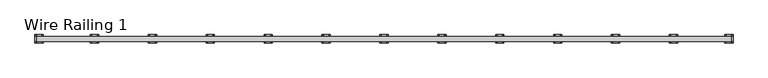
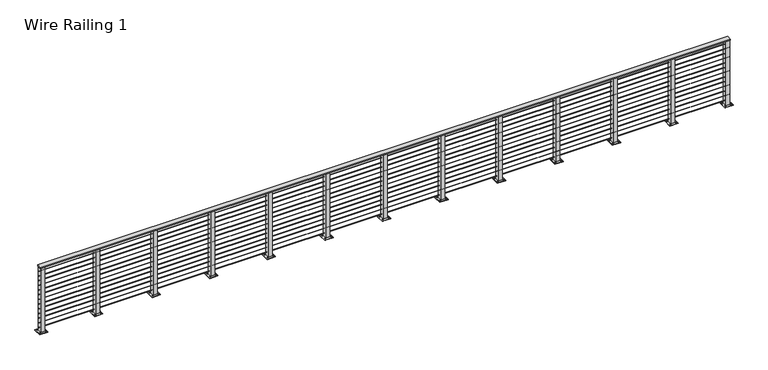
"""IFC4 building model written with IfcOpenShell, lengths in millimetres: railing geometry, Wire Railing 1."""

from ifc_helpers import new_model, si_unit, point, frame, frame_2d, origin, place, context, project, spatial, polyline, circle_curve, trimmed, segment, composite_curve, outline, extrude, source, transform, mapped, element, save


def wire_railing_1_673ce069(model_context):
    return source(origin(), model_context, "Body", "SweptSolid", [
        extrude(outline(polyline([(-281.8532828, -3023.5771465), (-281.8532828, -3099.7771465), (-10899.0532828, -3099.7771465), (-10899.0532828, -3023.5771465), (-281.8532828, -3023.5771465)])), frame((0.0, 0.0, 4502.15), z_axis=(0.0, 0.0, 1.0), x_axis=(1.0, 0.0, 0.0)), (0.0, 0.0, 1.0), 19.05),
        extrude(outline(composite_curve([segment(trimmed(circle_curve(frame_2d((-3061.6771465, 4442.61875)), 2.38125), [point((-3059.2958965, 4442.61875))], [point((-3064.0583965, 4442.61875))], False, "CARTESIAN"), True, "CONTINUOUS"), segment(trimmed(circle_curve(frame_2d((-3061.6771465, 4442.61875)), 2.38125), [point((-3064.0583965, 4442.61875))], [point((-3059.2958965, 4442.61875))], False, "CARTESIAN"), True, "CONTINUOUS")], self_intersect=False)), frame((-10899.0532828, 0.0, 0.0), z_axis=(1.0, 0.0, 0.0), x_axis=(0.0, 1.0, 0.0)), (0.0, 0.0, 1.0), 10617.2),
        extrude(outline(composite_curve([segment(trimmed(circle_curve(frame_2d((-3061.6771465, 4366.41875)), 2.38125), [point((-3059.2958965, 4366.41875))], [point((-3064.0583965, 4366.41875))], False, "CARTESIAN"), True, "CONTINUOUS"), segment(trimmed(circle_curve(frame_2d((-3061.6771465, 4366.41875)), 2.38125), [point((-3064.0583965, 4366.41875))], [point((-3059.2958965, 4366.41875))], False, "CARTESIAN"), True, "CONTINUOUS")], self_intersect=False)), frame((-10899.0532828, 0.0, 0.0), z_axis=(1.0, 0.0, 0.0), x_axis=(0.0, 1.0, 0.0)), (0.0, 0.0, 1.0), 10617.2),
        extrude(outline(composite_curve([segment(trimmed(circle_curve(frame_2d((-3061.6771465, 4290.21875)), 2.38125), [point((-3059.2958965, 4290.21875))], [point((-3064.0583965, 4290.21875))], False, "CARTESIAN"), True, "CONTINUOUS"), segment(trimmed(circle_curve(frame_2d((-3061.6771465, 4290.21875)), 2.38125), [point((-3064.0583965, 4290.21875))], [point((-3059.2958965, 4290.21875))], False, "CARTESIAN"), True, "CONTINUOUS")], self_intersect=False)), frame((-10899.0532828, 0.0, 0.0), z_axis=(1.0, 0.0, 0.0), x_axis=(0.0, 1.0, 0.0)), (0.0, 0.0, 1.0), 10617.2),
        extrude(outline(composite_curve([segment(trimmed(circle_curve(frame_2d((-3061.6771465, 4214.01875)), 2.38125), [point((-3059.2958965, 4214.01875))], [point((-3064.0583965, 4214.01875))], False, "CARTESIAN"), True, "CONTINUOUS"), segment(trimmed(circle_curve(frame_2d((-3061.6771465, 4214.01875)), 2.38125), [point((-3064.0583965, 4214.01875))], [point((-3059.2958965, 4214.01875))], False, "CARTESIAN"), True, "CONTINUOUS")], self_intersect=False)), frame((-10899.0532828, 0.0, 0.0), z_axis=(1.0, 0.0, 0.0), x_axis=(0.0, 1.0, 0.0)), (0.0, 0.0, 1.0), 10617.2),
        extrude(outline(composite_curve([segment(trimmed(circle_curve(frame_2d((-3061.6771465, 4137.81875)), 2.38125), [point((-3059.2958965, 4137.81875))], [point((-3064.0583965, 4137.81875))], False, "CARTESIAN"), True, "CONTINUOUS"), segment(trimmed(circle_curve(frame_2d((-3061.6771465, 4137.81875)), 2.38125), [point((-3064.0583965, 4137.81875))], [point((-3059.2958965, 4137.81875))], False, "CARTESIAN"), True, "CONTINUOUS")], self_intersect=False)), frame((-10899.0532828, 0.0, 0.0), z_axis=(1.0, 0.0, 0.0), x_axis=(0.0, 1.0, 0.0)), (0.0, 0.0, 1.0), 10617.2),
        extrude(outline(composite_curve([segment(trimmed(circle_curve(frame_2d((-3061.6771465, 4061.61875)), 2.38125), [point((-3059.2958965, 4061.61875))], [point((-3064.0583965, 4061.61875))], False, "CARTESIAN"), True, "CONTINUOUS"), segment(trimmed(circle_curve(frame_2d((-3061.6771465, 4061.61875)), 2.38125), [point((-3064.0583965, 4061.61875))], [point((-3059.2958965, 4061.61875))], False, "CARTESIAN"), True, "CONTINUOUS")], self_intersect=False)), frame((-10899.0532828, 0.0, 0.0), z_axis=(1.0, 0.0, 0.0), x_axis=(0.0, 1.0, 0.0)), (0.0, 0.0, 1.0), 10617.2),
        extrude(outline(composite_curve([segment(trimmed(circle_curve(frame_2d((-3061.6771465, 3985.41875)), 2.38125), [point((-3059.2958965, 3985.41875))], [point((-3064.0583965, 3985.41875))], False, "CARTESIAN"), True, "CONTINUOUS"), segment(trimmed(circle_curve(frame_2d((-3061.6771465, 3985.41875)), 2.38125), [point((-3064.0583965, 3985.41875))], [point((-3059.2958965, 3985.41875))], False, "CARTESIAN"), True, "CONTINUOUS")], self_intersect=False)), frame((-10899.0532828, 0.0, 0.0), z_axis=(1.0, 0.0, 0.0), x_axis=(0.0, 1.0, 0.0)), (0.0, 0.0, 1.0), 10617.2),
        extrude(outline(composite_curve([segment(trimmed(circle_curve(frame_2d((-3061.6771465, 3909.21875)), 2.38125), [point((-3059.2958965, 3909.21875))], [point((-3064.0583965, 3909.21875))], False, "CARTESIAN"), True, "CONTINUOUS"), segment(trimmed(circle_curve(frame_2d((-3061.6771465, 3909.21875)), 2.38125), [point((-3064.0583965, 3909.21875))], [point((-3059.2958965, 3909.21875))], False, "CARTESIAN"), True, "CONTINUOUS")], self_intersect=False)), frame((-10899.0532828, 0.0, 0.0), z_axis=(1.0, 0.0, 0.0), x_axis=(0.0, 1.0, 0.0)), (0.0, 0.0, 1.0), 10617.2),
        extrude(outline(composite_curve([segment(trimmed(circle_curve(frame_2d((-3061.6771465, 3833.01875)), 2.38125), [point((-3059.2958965, 3833.01875))], [point((-3064.0583965, 3833.01875))], False, "CARTESIAN"), True, "CONTINUOUS"), segment(trimmed(circle_curve(frame_2d((-3061.6771465, 3833.01875)), 2.38125), [point((-3064.0583965, 3833.01875))], [point((-3059.2958965, 3833.01875))], False, "CARTESIAN"), True, "CONTINUOUS")], self_intersect=False)), frame((-10899.0532828, 0.0, 0.0), z_axis=(1.0, 0.0, 0.0), x_axis=(0.0, 1.0, 0.0)), (0.0, 0.0, 1.0), 10617.2),
        extrude(outline(composite_curve([segment(trimmed(circle_curve(frame_2d((-3061.6771465, 3756.81875)), 2.38125), [point((-3059.2958965, 3756.81875))], [point((-3064.0583965, 3756.81875))], False, "CARTESIAN"), True, "CONTINUOUS"), segment(trimmed(circle_curve(frame_2d((-3061.6771465, 3756.81875)), 2.38125), [point((-3064.0583965, 3756.81875))], [point((-3059.2958965, 3756.81875))], False, "CARTESIAN"), True, "CONTINUOUS")], self_intersect=False)), frame((-10899.0532828, 0.0, 0.0), z_axis=(1.0, 0.0, 0.0), x_axis=(0.0, 1.0, 0.0)), (0.0, 0.0, 1.0), 10617.2),
        extrude(outline(composite_curve([segment(trimmed(circle_curve(frame_2d((-3061.6771465, 3680.61875)), 2.38125), [point((-3059.2958965, 3680.61875))], [point((-3064.0583965, 3680.61875))], False, "CARTESIAN"), True, "CONTINUOUS"), segment(trimmed(circle_curve(frame_2d((-3061.6771465, 3680.61875)), 2.38125), [point((-3064.0583965, 3680.61875))], [point((-3059.2958965, 3680.61875))], False, "CARTESIAN"), True, "CONTINUOUS")], self_intersect=False)), frame((-10899.0532828, 0.0, 0.0), z_axis=(1.0, 0.0, 0.0), x_axis=(0.0, 1.0, 0.0)), (0.0, 0.0, 1.0), 10617.2),
        extrude(outline(composite_curve([segment(trimmed(circle_curve(frame_2d((-3061.6771465, 3604.41875)), 2.38125), [point((-3059.2958965, 3604.41875))], [point((-3064.0583965, 3604.41875))], False, "CARTESIAN"), True, "CONTINUOUS"), segment(trimmed(circle_curve(frame_2d((-3061.6771465, 3604.41875)), 2.38125), [point((-3064.0583965, 3604.41875))], [point((-3059.2958965, 3604.41875))], False, "CARTESIAN"), True, "CONTINUOUS")], self_intersect=False)), frame((-10899.0532828, 0.0, 0.0), z_axis=(1.0, 0.0, 0.0), x_axis=(0.0, 1.0, 0.0)), (0.0, 0.0, 1.0), 10617.2),
        extrude(outline(composite_curve([segment(trimmed(circle_curve(frame_2d((-3061.6771465, 3528.21875)), 2.38125), [point((-3059.2958965, 3528.21875))], [point((-3064.0583965, 3528.21875))], False, "CARTESIAN"), True, "CONTINUOUS"), segment(trimmed(circle_curve(frame_2d((-3061.6771465, 3528.21875)), 2.38125), [point((-3064.0583965, 3528.21875))], [point((-3059.2958965, 3528.21875))], False, "CARTESIAN"), True, "CONTINUOUS")], self_intersect=False)), frame((-10899.0532828, 0.0, 0.0), z_axis=(1.0, 0.0, 0.0), x_axis=(0.0, 1.0, 0.0)), (0.0, 0.0, 1.0), 10617.2),
        extrude(outline(composite_curve([segment(trimmed(circle_curve(frame_2d((-9969.8366161, -3106.1271465)), 6.35), [point((-9969.8366161, -3112.4771465))], [point((-9969.8366161, -3099.7771465))], False, "CARTESIAN"), True, "CONTINUOUS"), segment(trimmed(circle_curve(frame_2d((-9969.8366161, -3106.1271465)), 6.35), [point((-9969.8366161, -3099.7771465))], [point((-9969.8366161, -3112.4771465))], False, "CARTESIAN"), True, "CONTINUOUS")], self_intersect=False)), frame((0.0, 0.0, 3454.4), z_axis=(0.0, 0.0, 1.0), x_axis=(1.0, 0.0, 0.0)), (0.0, 0.0, 1.0), 12.7),
        extrude(outline(composite_curve([segment(trimmed(circle_curve(frame_2d((-9969.8366161, -3017.2271465)), 6.35), [point((-9969.8366161, -3023.5771465))], [point((-9969.8366161, -3010.8771465))], False, "CARTESIAN"), True, "CONTINUOUS"), segment(trimmed(circle_curve(frame_2d((-9969.8366161, -3017.2271465)), 6.35), [point((-9969.8366161, -3010.8771465))], [point((-9969.8366161, -3023.5771465))], False, "CARTESIAN"), True, "CONTINUOUS")], self_intersect=False)), frame((0.0, 0.0, 3454.4), z_axis=(0.0, 0.0, 1.0), x_axis=(1.0, 0.0, 0.0)), (0.0, 0.0, 1.0), 12.7),
        extrude(outline(composite_curve([segment(trimmed(circle_curve(frame_2d((-10058.7366161, -3106.1271465)), 6.35), [point((-10058.7366161, -3112.4771465))], [point((-10058.7366161, -3099.7771465))], False, "CARTESIAN"), True, "CONTINUOUS"), segment(trimmed(circle_curve(frame_2d((-10058.7366161, -3106.1271465)), 6.35), [point((-10058.7366161, -3099.7771465))], [point((-10058.7366161, -3112.4771465))], False, "CARTESIAN"), True, "CONTINUOUS")], self_intersect=False)), frame((0.0, 0.0, 3454.4), z_axis=(0.0, 0.0, 1.0), x_axis=(1.0, 0.0, 0.0)), (0.0, 0.0, 1.0), 12.7),
        extrude(outline(composite_curve([segment(trimmed(circle_curve(frame_2d((-10058.7366161, -3017.2271465)), 6.35), [point((-10058.7366161, -3023.5771465))], [point((-10058.7366161, -3010.8771465))], False, "CARTESIAN"), True, "CONTINUOUS"), segment(trimmed(circle_curve(frame_2d((-10058.7366161, -3017.2271465)), 6.35), [point((-10058.7366161, -3010.8771465))], [point((-10058.7366161, -3023.5771465))], False, "CARTESIAN"), True, "CONTINUOUS")], self_intersect=False)), frame((0.0, 0.0, 3454.4), z_axis=(0.0, 0.0, 1.0), x_axis=(1.0, 0.0, 0.0)), (0.0, 0.0, 1.0), 12.7),
        extrude(outline(polyline([(-9950.7866161, -2998.1771465), (-9950.7866161, -3125.1771465), (-10077.7866161, -3125.1771465), (-10077.7866161, -2998.1771465), (-9950.7866161, -2998.1771465)])), frame((0.0, 0.0, 3454.4), z_axis=(0.0, 0.0, 1.0), x_axis=(1.0, 0.0, 0.0)), (0.0, 0.0, 1.0), 6.35),
        extrude(outline(polyline([(-9984.1241161, -3031.5146465), (-9984.1241161, -3091.8396465), (-10044.4491161, -3091.8396465), (-10044.4491161, -3031.5146465), (-9984.1241161, -3031.5146465)]), holes=[polyline([(-9990.4741161, -3037.8646465), (-10038.0991161, -3037.8646465), (-10038.0991161, -3085.4896465), (-9990.4741161, -3085.4896465), (-9990.4741161, -3037.8646465)])]), frame((0.0, 0.0, 3454.4), z_axis=(0.0, 0.0, 1.0), x_axis=(1.0, 0.0, 0.0)), (0.0, 0.0, 1.0), 1047.75),
        extrude(outline(composite_curve([segment(trimmed(circle_curve(frame_2d((-9085.0699495, -3106.1271465)), 6.35), [point((-9085.0699495, -3112.4771465))], [point((-9085.0699495, -3099.7771465))], False, "CARTESIAN"), True, "CONTINUOUS"), segment(trimmed(circle_curve(frame_2d((-9085.0699495, -3106.1271465)), 6.35), [point((-9085.0699495, -3099.7771465))], [point((-9085.0699495, -3112.4771465))], False, "CARTESIAN"), True, "CONTINUOUS")], self_intersect=False)), frame((0.0, 0.0, 3454.4), z_axis=(0.0, 0.0, 1.0), x_axis=(1.0, 0.0, 0.0)), (0.0, 0.0, 1.0), 12.7),
        extrude(outline(composite_curve([segment(trimmed(circle_curve(frame_2d((-9085.0699495, -3017.2271465)), 6.35), [point((-9085.0699495, -3023.5771465))], [point((-9085.0699495, -3010.8771465))], False, "CARTESIAN"), True, "CONTINUOUS"), segment(trimmed(circle_curve(frame_2d((-9085.0699495, -3017.2271465)), 6.35), [point((-9085.0699495, -3010.8771465))], [point((-9085.0699495, -3023.5771465))], False, "CARTESIAN"), True, "CONTINUOUS")], self_intersect=False)), frame((0.0, 0.0, 3454.4), z_axis=(0.0, 0.0, 1.0), x_axis=(1.0, 0.0, 0.0)), (0.0, 0.0, 1.0), 12.7),
        extrude(outline(composite_curve([segment(trimmed(circle_curve(frame_2d((-9173.9699495, -3106.1271465)), 6.35), [point((-9173.9699495, -3112.4771465))], [point((-9173.9699495, -3099.7771465))], False, "CARTESIAN"), True, "CONTINUOUS"), segment(trimmed(circle_curve(frame_2d((-9173.9699495, -3106.1271465)), 6.35), [point((-9173.9699495, -3099.7771465))], [point((-9173.9699495, -3112.4771465))], False, "CARTESIAN"), True, "CONTINUOUS")], self_intersect=False)), frame((0.0, 0.0, 3454.4), z_axis=(0.0, 0.0, 1.0), x_axis=(1.0, 0.0, 0.0)), (0.0, 0.0, 1.0), 12.7),
        extrude(outline(composite_curve([segment(trimmed(circle_curve(frame_2d((-9173.9699495, -3017.2271465)), 6.35), [point((-9173.9699495, -3023.5771465))], [point((-9173.9699495, -3010.8771465))], False, "CARTESIAN"), True, "CONTINUOUS"), segment(trimmed(circle_curve(frame_2d((-9173.9699495, -3017.2271465)), 6.35), [point((-9173.9699495, -3010.8771465))], [point((-9173.9699495, -3023.5771465))], False, "CARTESIAN"), True, "CONTINUOUS")], self_intersect=False)), frame((0.0, 0.0, 3454.4), z_axis=(0.0, 0.0, 1.0), x_axis=(1.0, 0.0, 0.0)), (0.0, 0.0, 1.0), 12.7),
        extrude(outline(polyline([(-9066.0199495, -2998.1771465), (-9066.0199495, -3125.1771465), (-9193.0199495, -3125.1771465), (-9193.0199495, -2998.1771465), (-9066.0199495, -2998.1771465)])), frame((0.0, 0.0, 3454.4), z_axis=(0.0, 0.0, 1.0), x_axis=(1.0, 0.0, 0.0)), (0.0, 0.0, 1.0), 6.35),
        extrude(outline(polyline([(-9099.3574495, -3031.5146465), (-9099.3574495, -3091.8396465), (-9159.6824495, -3091.8396465), (-9159.6824495, -3031.5146465), (-9099.3574495, -3031.5146465)]), holes=[polyline([(-9105.7074495, -3037.8646465), (-9153.3324495, -3037.8646465), (-9153.3324495, -3085.4896465), (-9105.7074495, -3085.4896465), (-9105.7074495, -3037.8646465)])]), frame((0.0, 0.0, 3454.4), z_axis=(0.0, 0.0, 1.0), x_axis=(1.0, 0.0, 0.0)), (0.0, 0.0, 1.0), 1047.75),
        extrude(outline(composite_curve([segment(trimmed(circle_curve(frame_2d((-8200.3032828, -3106.1271465)), 6.35), [point((-8200.3032828, -3112.4771465))], [point((-8200.3032828, -3099.7771465))], False, "CARTESIAN"), True, "CONTINUOUS"), segment(trimmed(circle_curve(frame_2d((-8200.3032828, -3106.1271465)), 6.35), [point((-8200.3032828, -3099.7771465))], [point((-8200.3032828, -3112.4771465))], False, "CARTESIAN"), True, "CONTINUOUS")], self_intersect=False)), frame((0.0, 0.0, 3454.4), z_axis=(0.0, 0.0, 1.0), x_axis=(1.0, 0.0, 0.0)), (0.0, 0.0, 1.0), 12.7),
        extrude(outline(composite_curve([segment(trimmed(circle_curve(frame_2d((-8200.3032828, -3017.2271465)), 6.35), [point((-8200.3032828, -3023.5771465))], [point((-8200.3032828, -3010.8771465))], False, "CARTESIAN"), True, "CONTINUOUS"), segment(trimmed(circle_curve(frame_2d((-8200.3032828, -3017.2271465)), 6.35), [point((-8200.3032828, -3010.8771465))], [point((-8200.3032828, -3023.5771465))], False, "CARTESIAN"), True, "CONTINUOUS")], self_intersect=False)), frame((0.0, 0.0, 3454.4), z_axis=(0.0, 0.0, 1.0), x_axis=(1.0, 0.0, 0.0)), (0.0, 0.0, 1.0), 12.7),
        extrude(outline(composite_curve([segment(trimmed(circle_curve(frame_2d((-8289.2032828, -3106.1271465)), 6.35), [point((-8289.2032828, -3112.4771465))], [point((-8289.2032828, -3099.7771465))], False, "CARTESIAN"), True, "CONTINUOUS"), segment(trimmed(circle_curve(frame_2d((-8289.2032828, -3106.1271465)), 6.35), [point((-8289.2032828, -3099.7771465))], [point((-8289.2032828, -3112.4771465))], False, "CARTESIAN"), True, "CONTINUOUS")], self_intersect=False)), frame((0.0, 0.0, 3454.4), z_axis=(0.0, 0.0, 1.0), x_axis=(1.0, 0.0, 0.0)), (0.0, 0.0, 1.0), 12.7),
        extrude(outline(composite_curve([segment(trimmed(circle_curve(frame_2d((-8289.2032828, -3017.2271465)), 6.35), [point((-8289.2032828, -3023.5771465))], [point((-8289.2032828, -3010.8771465))], False, "CARTESIAN"), True, "CONTINUOUS"), segment(trimmed(circle_curve(frame_2d((-8289.2032828, -3017.2271465)), 6.35), [point((-8289.2032828, -3010.8771465))], [point((-8289.2032828, -3023.5771465))], False, "CARTESIAN"), True, "CONTINUOUS")], self_intersect=False)), frame((0.0, 0.0, 3454.4), z_axis=(0.0, 0.0, 1.0), x_axis=(1.0, 0.0, 0.0)), (0.0, 0.0, 1.0), 12.7),
        extrude(outline(polyline([(-8181.2532828, -2998.1771465), (-8181.2532828, -3125.1771465), (-8308.2532828, -3125.1771465), (-8308.2532828, -2998.1771465), (-8181.2532828, -2998.1771465)])), frame((0.0, 0.0, 3454.4), z_axis=(0.0, 0.0, 1.0), x_axis=(1.0, 0.0, 0.0)), (0.0, 0.0, 1.0), 6.35),
        extrude(outline(polyline([(-8214.5907828, -3031.5146465), (-8214.5907828, -3091.8396465), (-8274.9157828, -3091.8396465), (-8274.9157828, -3031.5146465), (-8214.5907828, -3031.5146465)]), holes=[polyline([(-8220.9407828, -3037.8646465), (-8268.5657828, -3037.8646465), (-8268.5657828, -3085.4896465), (-8220.9407828, -3085.4896465), (-8220.9407828, -3037.8646465)])]), frame((0.0, 0.0, 3454.4), z_axis=(0.0, 0.0, 1.0), x_axis=(1.0, 0.0, 0.0)), (0.0, 0.0, 1.0), 1047.75),
        extrude(outline(composite_curve([segment(trimmed(circle_curve(frame_2d((-7315.5366161, -3106.1271465)), 6.35), [point((-7315.5366161, -3112.4771465))], [point((-7315.5366161, -3099.7771465))], False, "CARTESIAN"), True, "CONTINUOUS"), segment(trimmed(circle_curve(frame_2d((-7315.5366161, -3106.1271465)), 6.35), [point((-7315.5366161, -3099.7771465))], [point((-7315.5366161, -3112.4771465))], False, "CARTESIAN"), True, "CONTINUOUS")], self_intersect=False)), frame((0.0, 0.0, 3454.4), z_axis=(0.0, 0.0, 1.0), x_axis=(1.0, 0.0, 0.0)), (0.0, 0.0, 1.0), 12.7),
        extrude(outline(composite_curve([segment(trimmed(circle_curve(frame_2d((-7315.5366161, -3017.2271465)), 6.35), [point((-7315.5366161, -3023.5771465))], [point((-7315.5366161, -3010.8771465))], False, "CARTESIAN"), True, "CONTINUOUS"), segment(trimmed(circle_curve(frame_2d((-7315.5366161, -3017.2271465)), 6.35), [point((-7315.5366161, -3010.8771465))], [point((-7315.5366161, -3023.5771465))], False, "CARTESIAN"), True, "CONTINUOUS")], self_intersect=False)), frame((0.0, 0.0, 3454.4), z_axis=(0.0, 0.0, 1.0), x_axis=(1.0, 0.0, 0.0)), (0.0, 0.0, 1.0), 12.7),
        extrude(outline(composite_curve([segment(trimmed(circle_curve(frame_2d((-7404.4366161, -3106.1271465)), 6.35), [point((-7404.4366161, -3112.4771465))], [point((-7404.4366161, -3099.7771465))], False, "CARTESIAN"), True, "CONTINUOUS"), segment(trimmed(circle_curve(frame_2d((-7404.4366161, -3106.1271465)), 6.35), [point((-7404.4366161, -3099.7771465))], [point((-7404.4366161, -3112.4771465))], False, "CARTESIAN"), True, "CONTINUOUS")], self_intersect=False)), frame((0.0, 0.0, 3454.4), z_axis=(0.0, 0.0, 1.0), x_axis=(1.0, 0.0, 0.0)), (0.0, 0.0, 1.0), 12.7),
        extrude(outline(composite_curve([segment(trimmed(circle_curve(frame_2d((-7404.4366161, -3017.2271465)), 6.35), [point((-7404.4366161, -3023.5771465))], [point((-7404.4366161, -3010.8771465))], False, "CARTESIAN"), True, "CONTINUOUS"), segment(trimmed(circle_curve(frame_2d((-7404.4366161, -3017.2271465)), 6.35), [point((-7404.4366161, -3010.8771465))], [point((-7404.4366161, -3023.5771465))], False, "CARTESIAN"), True, "CONTINUOUS")], self_intersect=False)), frame((0.0, 0.0, 3454.4), z_axis=(0.0, 0.0, 1.0), x_axis=(1.0, 0.0, 0.0)), (0.0, 0.0, 1.0), 12.7),
        extrude(outline(polyline([(-7296.4866161, -2998.1771465), (-7296.4866161, -3125.1771465), (-7423.4866161, -3125.1771465), (-7423.4866161, -2998.1771465), (-7296.4866161, -2998.1771465)])), frame((0.0, 0.0, 3454.4), z_axis=(0.0, 0.0, 1.0), x_axis=(1.0, 0.0, 0.0)), (0.0, 0.0, 1.0), 6.35),
        extrude(outline(polyline([(-7329.8241161, -3031.5146465), (-7329.8241161, -3091.8396465), (-7390.1491161, -3091.8396465), (-7390.1491161, -3031.5146465), (-7329.8241161, -3031.5146465)]), holes=[polyline([(-7336.1741161, -3037.8646465), (-7383.7991161, -3037.8646465), (-7383.7991161, -3085.4896465), (-7336.1741161, -3085.4896465), (-7336.1741161, -3037.8646465)])]), frame((0.0, 0.0, 3454.4), z_axis=(0.0, 0.0, 1.0), x_axis=(1.0, 0.0, 0.0)), (0.0, 0.0, 1.0), 1047.75),
        extrude(outline(composite_curve([segment(trimmed(circle_curve(frame_2d((-6430.7699495, -3106.1271465)), 6.35), [point((-6430.7699495, -3112.4771465))], [point((-6430.7699495, -3099.7771465))], False, "CARTESIAN"), True, "CONTINUOUS"), segment(trimmed(circle_curve(frame_2d((-6430.7699495, -3106.1271465)), 6.35), [point((-6430.7699495, -3099.7771465))], [point((-6430.7699495, -3112.4771465))], False, "CARTESIAN"), True, "CONTINUOUS")], self_intersect=False)), frame((0.0, 0.0, 3454.4), z_axis=(0.0, 0.0, 1.0), x_axis=(1.0, 0.0, 0.0)), (0.0, 0.0, 1.0), 12.7),
        extrude(outline(composite_curve([segment(trimmed(circle_curve(frame_2d((-6430.7699495, -3017.2271465)), 6.35), [point((-6430.7699495, -3023.5771465))], [point((-6430.7699495, -3010.8771465))], False, "CARTESIAN"), True, "CONTINUOUS"), segment(trimmed(circle_curve(frame_2d((-6430.7699495, -3017.2271465)), 6.35), [point((-6430.7699495, -3010.8771465))], [point((-6430.7699495, -3023.5771465))], False, "CARTESIAN"), True, "CONTINUOUS")], self_intersect=False)), frame((0.0, 0.0, 3454.4), z_axis=(0.0, 0.0, 1.0), x_axis=(1.0, 0.0, 0.0)), (0.0, 0.0, 1.0), 12.7),
        extrude(outline(composite_curve([segment(trimmed(circle_curve(frame_2d((-6519.6699495, -3106.1271465)), 6.35), [point((-6519.6699495, -3112.4771465))], [point((-6519.6699495, -3099.7771465))], False, "CARTESIAN"), True, "CONTINUOUS"), segment(trimmed(circle_curve(frame_2d((-6519.6699495, -3106.1271465)), 6.35), [point((-6519.6699495, -3099.7771465))], [point((-6519.6699495, -3112.4771465))], False, "CARTESIAN"), True, "CONTINUOUS")], self_intersect=False)), frame((0.0, 0.0, 3454.4), z_axis=(0.0, 0.0, 1.0), x_axis=(1.0, 0.0, 0.0)), (0.0, 0.0, 1.0), 12.7),
        extrude(outline(composite_curve([segment(trimmed(circle_curve(frame_2d((-6519.6699495, -3017.2271465)), 6.35), [point((-6519.6699495, -3023.5771465))], [point((-6519.6699495, -3010.8771465))], False, "CARTESIAN"), True, "CONTINUOUS"), segment(trimmed(circle_curve(frame_2d((-6519.6699495, -3017.2271465)), 6.35), [point((-6519.6699495, -3010.8771465))], [point((-6519.6699495, -3023.5771465))], False, "CARTESIAN"), True, "CONTINUOUS")], self_intersect=False)), frame((0.0, 0.0, 3454.4), z_axis=(0.0, 0.0, 1.0), x_axis=(1.0, 0.0, 0.0)), (0.0, 0.0, 1.0), 12.7),
        extrude(outline(polyline([(-6411.7199495, -2998.1771465), (-6411.7199495, -3125.1771465), (-6538.7199495, -3125.1771465), (-6538.7199495, -2998.1771465), (-6411.7199495, -2998.1771465)])), frame((0.0, 0.0, 3454.4), z_axis=(0.0, 0.0, 1.0), x_axis=(1.0, 0.0, 0.0)), (0.0, 0.0, 1.0), 6.35),
        extrude(outline(polyline([(-6445.0574495, -3031.5146465), (-6445.0574495, -3091.8396465), (-6505.3824495, -3091.8396465), (-6505.3824495, -3031.5146465), (-6445.0574495, -3031.5146465)]), holes=[polyline([(-6451.4074495, -3037.8646465), (-6499.0324495, -3037.8646465), (-6499.0324495, -3085.4896465), (-6451.4074495, -3085.4896465), (-6451.4074495, -3037.8646465)])]), frame((0.0, 0.0, 3454.4), z_axis=(0.0, 0.0, 1.0), x_axis=(1.0, 0.0, 0.0)), (0.0, 0.0, 1.0), 1047.75),
        extrude(outline(composite_curve([segment(trimmed(circle_curve(frame_2d((-5546.0032828, -3106.1271465)), 6.35), [point((-5546.0032828, -3112.4771465))], [point((-5546.0032828, -3099.7771465))], False, "CARTESIAN"), True, "CONTINUOUS"), segment(trimmed(circle_curve(frame_2d((-5546.0032828, -3106.1271465)), 6.35), [point((-5546.0032828, -3099.7771465))], [point((-5546.0032828, -3112.4771465))], False, "CARTESIAN"), True, "CONTINUOUS")], self_intersect=False)), frame((0.0, 0.0, 3454.4), z_axis=(0.0, 0.0, 1.0), x_axis=(1.0, 0.0, 0.0)), (0.0, 0.0, 1.0), 12.7),
        extrude(outline(composite_curve([segment(trimmed(circle_curve(frame_2d((-5546.0032828, -3017.2271465)), 6.35), [point((-5546.0032828, -3023.5771465))], [point((-5546.0032828, -3010.8771465))], False, "CARTESIAN"), True, "CONTINUOUS"), segment(trimmed(circle_curve(frame_2d((-5546.0032828, -3017.2271465)), 6.35), [point((-5546.0032828, -3010.8771465))], [point((-5546.0032828, -3023.5771465))], False, "CARTESIAN"), True, "CONTINUOUS")], self_intersect=False)), frame((0.0, 0.0, 3454.4), z_axis=(0.0, 0.0, 1.0), x_axis=(1.0, 0.0, 0.0)), (0.0, 0.0, 1.0), 12.7),
        extrude(outline(composite_curve([segment(trimmed(circle_curve(frame_2d((-5634.9032828, -3106.1271465)), 6.35), [point((-5634.9032828, -3112.4771465))], [point((-5634.9032828, -3099.7771465))], False, "CARTESIAN"), True, "CONTINUOUS"), segment(trimmed(circle_curve(frame_2d((-5634.9032828, -3106.1271465)), 6.35), [point((-5634.9032828, -3099.7771465))], [point((-5634.9032828, -3112.4771465))], False, "CARTESIAN"), True, "CONTINUOUS")], self_intersect=False)), frame((0.0, 0.0, 3454.4), z_axis=(0.0, 0.0, 1.0), x_axis=(1.0, 0.0, 0.0)), (0.0, 0.0, 1.0), 12.7),
        extrude(outline(composite_curve([segment(trimmed(circle_curve(frame_2d((-5634.9032828, -3017.2271465)), 6.35), [point((-5634.9032828, -3023.5771465))], [point((-5634.9032828, -3010.8771465))], False, "CARTESIAN"), True, "CONTINUOUS"), segment(trimmed(circle_curve(frame_2d((-5634.9032828, -3017.2271465)), 6.35), [point((-5634.9032828, -3010.8771465))], [point((-5634.9032828, -3023.5771465))], False, "CARTESIAN"), True, "CONTINUOUS")], self_intersect=False)), frame((0.0, 0.0, 3454.4), z_axis=(0.0, 0.0, 1.0), x_axis=(1.0, 0.0, 0.0)), (0.0, 0.0, 1.0), 12.7),
        extrude(outline(polyline([(-5526.9532828, -2998.1771465), (-5526.9532828, -3125.1771465), (-5653.9532828, -3125.1771465), (-5653.9532828, -2998.1771465), (-5526.9532828, -2998.1771465)])), frame((0.0, 0.0, 3454.4), z_axis=(0.0, 0.0, 1.0), x_axis=(1.0, 0.0, 0.0)), (0.0, 0.0, 1.0), 6.35),
        extrude(outline(polyline([(-5560.2907828, -3031.5146465), (-5560.2907828, -3091.8396465), (-5620.6157828, -3091.8396465), (-5620.6157828, -3031.5146465), (-5560.2907828, -3031.5146465)]), holes=[polyline([(-5566.6407828, -3037.8646465), (-5614.2657828, -3037.8646465), (-5614.2657828, -3085.4896465), (-5566.6407828, -3085.4896465), (-5566.6407828, -3037.8646465)])]), frame((0.0, 0.0, 3454.4), z_axis=(0.0, 0.0, 1.0), x_axis=(1.0, 0.0, 0.0)), (0.0, 0.0, 1.0), 1047.75),
        extrude(outline(composite_curve([segment(trimmed(circle_curve(frame_2d((-4661.2366161, -3106.1271465)), 6.35), [point((-4661.2366161, -3112.4771465))], [point((-4661.2366161, -3099.7771465))], False, "CARTESIAN"), True, "CONTINUOUS"), segment(trimmed(circle_curve(frame_2d((-4661.2366161, -3106.1271465)), 6.35), [point((-4661.2366161, -3099.7771465))], [point((-4661.2366161, -3112.4771465))], False, "CARTESIAN"), True, "CONTINUOUS")], self_intersect=False)), frame((0.0, 0.0, 3454.4), z_axis=(0.0, 0.0, 1.0), x_axis=(1.0, 0.0, 0.0)), (0.0, 0.0, 1.0), 12.7),
        extrude(outline(composite_curve([segment(trimmed(circle_curve(frame_2d((-4661.2366161, -3017.2271465)), 6.35), [point((-4661.2366161, -3023.5771465))], [point((-4661.2366161, -3010.8771465))], False, "CARTESIAN"), True, "CONTINUOUS"), segment(trimmed(circle_curve(frame_2d((-4661.2366161, -3017.2271465)), 6.35), [point((-4661.2366161, -3010.8771465))], [point((-4661.2366161, -3023.5771465))], False, "CARTESIAN"), True, "CONTINUOUS")], self_intersect=False)), frame((0.0, 0.0, 3454.4), z_axis=(0.0, 0.0, 1.0), x_axis=(1.0, 0.0, 0.0)), (0.0, 0.0, 1.0), 12.7),
        extrude(outline(composite_curve([segment(trimmed(circle_curve(frame_2d((-4750.1366161, -3106.1271465)), 6.35), [point((-4750.1366161, -3112.4771465))], [point((-4750.1366161, -3099.7771465))], False, "CARTESIAN"), True, "CONTINUOUS"), segment(trimmed(circle_curve(frame_2d((-4750.1366161, -3106.1271465)), 6.35), [point((-4750.1366161, -3099.7771465))], [point((-4750.1366161, -3112.4771465))], False, "CARTESIAN"), True, "CONTINUOUS")], self_intersect=False)), frame((0.0, 0.0, 3454.4), z_axis=(0.0, 0.0, 1.0), x_axis=(1.0, 0.0, 0.0)), (0.0, 0.0, 1.0), 12.7),
        extrude(outline(composite_curve([segment(trimmed(circle_curve(frame_2d((-4750.1366161, -3017.2271465)), 6.35), [point((-4750.1366161, -3023.5771465))], [point((-4750.1366161, -3010.8771465))], False, "CARTESIAN"), True, "CONTINUOUS"), segment(trimmed(circle_curve(frame_2d((-4750.1366161, -3017.2271465)), 6.35), [point((-4750.1366161, -3010.8771465))], [point((-4750.1366161, -3023.5771465))], False, "CARTESIAN"), True, "CONTINUOUS")], self_intersect=False)), frame((0.0, 0.0, 3454.4), z_axis=(0.0, 0.0, 1.0), x_axis=(1.0, 0.0, 0.0)), (0.0, 0.0, 1.0), 12.7),
        extrude(outline(polyline([(-4642.1866161, -2998.1771465), (-4642.1866161, -3125.1771465), (-4769.1866161, -3125.1771465), (-4769.1866161, -2998.1771465), (-4642.1866161, -2998.1771465)])), frame((0.0, 0.0, 3454.4), z_axis=(0.0, 0.0, 1.0), x_axis=(1.0, 0.0, 0.0)), (0.0, 0.0, 1.0), 6.35),
        extrude(outline(polyline([(-4675.5241161, -3031.5146465), (-4675.5241161, -3091.8396465), (-4735.8491161, -3091.8396465), (-4735.8491161, -3031.5146465), (-4675.5241161, -3031.5146465)]), holes=[polyline([(-4681.8741161, -3037.8646465), (-4729.4991161, -3037.8646465), (-4729.4991161, -3085.4896465), (-4681.8741161, -3085.4896465), (-4681.8741161, -3037.8646465)])]), frame((0.0, 0.0, 3454.4), z_axis=(0.0, 0.0, 1.0), x_axis=(1.0, 0.0, 0.0)), (0.0, 0.0, 1.0), 1047.75),
        extrude(outline(composite_curve([segment(trimmed(circle_curve(frame_2d((-3776.4699495, -3106.1271465)), 6.35), [point((-3776.4699495, -3112.4771465))], [point((-3776.4699495, -3099.7771465))], False, "CARTESIAN"), True, "CONTINUOUS"), segment(trimmed(circle_curve(frame_2d((-3776.4699495, -3106.1271465)), 6.35), [point((-3776.4699495, -3099.7771465))], [point((-3776.4699495, -3112.4771465))], False, "CARTESIAN"), True, "CONTINUOUS")], self_intersect=False)), frame((0.0, 0.0, 3454.4), z_axis=(0.0, 0.0, 1.0), x_axis=(1.0, 0.0, 0.0)), (0.0, 0.0, 1.0), 12.7),
        extrude(outline(composite_curve([segment(trimmed(circle_curve(frame_2d((-3776.4699495, -3017.2271465)), 6.35), [point((-3776.4699495, -3023.5771465))], [point((-3776.4699495, -3010.8771465))], False, "CARTESIAN"), True, "CONTINUOUS"), segment(trimmed(circle_curve(frame_2d((-3776.4699495, -3017.2271465)), 6.35), [point((-3776.4699495, -3010.8771465))], [point((-3776.4699495, -3023.5771465))], False, "CARTESIAN"), True, "CONTINUOUS")], self_intersect=False)), frame((0.0, 0.0, 3454.4), z_axis=(0.0, 0.0, 1.0), x_axis=(1.0, 0.0, 0.0)), (0.0, 0.0, 1.0), 12.7),
        extrude(outline(composite_curve([segment(trimmed(circle_curve(frame_2d((-3865.3699495, -3106.1271465)), 6.35), [point((-3865.3699495, -3112.4771465))], [point((-3865.3699495, -3099.7771465))], False, "CARTESIAN"), True, "CONTINUOUS"), segment(trimmed(circle_curve(frame_2d((-3865.3699495, -3106.1271465)), 6.35), [point((-3865.3699495, -3099.7771465))], [point((-3865.3699495, -3112.4771465))], False, "CARTESIAN"), True, "CONTINUOUS")], self_intersect=False)), frame((0.0, 0.0, 3454.4), z_axis=(0.0, 0.0, 1.0), x_axis=(1.0, 0.0, 0.0)), (0.0, 0.0, 1.0), 12.7),
        extrude(outline(composite_curve([segment(trimmed(circle_curve(frame_2d((-3865.3699495, -3017.2271465)), 6.35), [point((-3865.3699495, -3023.5771465))], [point((-3865.3699495, -3010.8771465))], False, "CARTESIAN"), True, "CONTINUOUS"), segment(trimmed(circle_curve(frame_2d((-3865.3699495, -3017.2271465)), 6.35), [point((-3865.3699495, -3010.8771465))], [point((-3865.3699495, -3023.5771465))], False, "CARTESIAN"), True, "CONTINUOUS")], self_intersect=False)), frame((0.0, 0.0, 3454.4), z_axis=(0.0, 0.0, 1.0), x_axis=(1.0, 0.0, 0.0)), (0.0, 0.0, 1.0), 12.7),
        extrude(outline(polyline([(-3757.4199495, -2998.1771465), (-3757.4199495, -3125.1771465), (-3884.4199495, -3125.1771465), (-3884.4199495, -2998.1771465), (-3757.4199495, -2998.1771465)])), frame((0.0, 0.0, 3454.4), z_axis=(0.0, 0.0, 1.0), x_axis=(1.0, 0.0, 0.0)), (0.0, 0.0, 1.0), 6.35),
        extrude(outline(polyline([(-3790.7574495, -3031.5146465), (-3790.7574495, -3091.8396465), (-3851.0824495, -3091.8396465), (-3851.0824495, -3031.5146465), (-3790.7574495, -3031.5146465)]), holes=[polyline([(-3797.1074495, -3037.8646465), (-3844.7324495, -3037.8646465), (-3844.7324495, -3085.4896465), (-3797.1074495, -3085.4896465), (-3797.1074495, -3037.8646465)])]), frame((0.0, 0.0, 3454.4), z_axis=(0.0, 0.0, 1.0), x_axis=(1.0, 0.0, 0.0)), (0.0, 0.0, 1.0), 1047.75),
        extrude(outline(composite_curve([segment(trimmed(circle_curve(frame_2d((-2891.7032828, -3106.1271465)), 6.35), [point((-2891.7032828, -3112.4771465))], [point((-2891.7032828, -3099.7771465))], False, "CARTESIAN"), True, "CONTINUOUS"), segment(trimmed(circle_curve(frame_2d((-2891.7032828, -3106.1271465)), 6.35), [point((-2891.7032828, -3099.7771465))], [point((-2891.7032828, -3112.4771465))], False, "CARTESIAN"), True, "CONTINUOUS")], self_intersect=False)), frame((0.0, 0.0, 3454.4), z_axis=(0.0, 0.0, 1.0), x_axis=(1.0, 0.0, 0.0)), (0.0, 0.0, 1.0), 12.7),
        extrude(outline(composite_curve([segment(trimmed(circle_curve(frame_2d((-2891.7032828, -3017.2271465)), 6.35), [point((-2891.7032828, -3023.5771465))], [point((-2891.7032828, -3010.8771465))], False, "CARTESIAN"), True, "CONTINUOUS"), segment(trimmed(circle_curve(frame_2d((-2891.7032828, -3017.2271465)), 6.35), [point((-2891.7032828, -3010.8771465))], [point((-2891.7032828, -3023.5771465))], False, "CARTESIAN"), True, "CONTINUOUS")], self_intersect=False)), frame((0.0, 0.0, 3454.4), z_axis=(0.0, 0.0, 1.0), x_axis=(1.0, 0.0, 0.0)), (0.0, 0.0, 1.0), 12.7),
        extrude(outline(composite_curve([segment(trimmed(circle_curve(frame_2d((-2980.6032828, -3106.1271465)), 6.35), [point((-2980.6032828, -3112.4771465))], [point((-2980.6032828, -3099.7771465))], False, "CARTESIAN"), True, "CONTINUOUS"), segment(trimmed(circle_curve(frame_2d((-2980.6032828, -3106.1271465)), 6.35), [point((-2980.6032828, -3099.7771465))], [point((-2980.6032828, -3112.4771465))], False, "CARTESIAN"), True, "CONTINUOUS")], self_intersect=False)), frame((0.0, 0.0, 3454.4), z_axis=(0.0, 0.0, 1.0), x_axis=(1.0, 0.0, 0.0)), (0.0, 0.0, 1.0), 12.7),
        extrude(outline(composite_curve([segment(trimmed(circle_curve(frame_2d((-2980.6032828, -3017.2271465)), 6.35), [point((-2980.6032828, -3023.5771465))], [point((-2980.6032828, -3010.8771465))], False, "CARTESIAN"), True, "CONTINUOUS"), segment(trimmed(circle_curve(frame_2d((-2980.6032828, -3017.2271465)), 6.35), [point((-2980.6032828, -3010.8771465))], [point((-2980.6032828, -3023.5771465))], False, "CARTESIAN"), True, "CONTINUOUS")], self_intersect=False)), frame((0.0, 0.0, 3454.4), z_axis=(0.0, 0.0, 1.0), x_axis=(1.0, 0.0, 0.0)), (0.0, 0.0, 1.0), 12.7),
        extrude(outline(polyline([(-2872.6532828, -2998.1771465), (-2872.6532828, -3125.1771465), (-2999.6532828, -3125.1771465), (-2999.6532828, -2998.1771465), (-2872.6532828, -2998.1771465)])), frame((0.0, 0.0, 3454.4), z_axis=(0.0, 0.0, 1.0), x_axis=(1.0, 0.0, 0.0)), (0.0, 0.0, 1.0), 6.35),
        extrude(outline(polyline([(-2905.9907828, -3031.5146465), (-2905.9907828, -3091.8396465), (-2966.3157828, -3091.8396465), (-2966.3157828, -3031.5146465), (-2905.9907828, -3031.5146465)]), holes=[polyline([(-2912.3407828, -3037.8646465), (-2959.9657828, -3037.8646465), (-2959.9657828, -3085.4896465), (-2912.3407828, -3085.4896465), (-2912.3407828, -3037.8646465)])]), frame((0.0, 0.0, 3454.4), z_axis=(0.0, 0.0, 1.0), x_axis=(1.0, 0.0, 0.0)), (0.0, 0.0, 1.0), 1047.75),
        extrude(outline(composite_curve([segment(trimmed(circle_curve(frame_2d((-2006.9366161, -3106.1271465)), 6.35), [point((-2006.9366161, -3112.4771465))], [point((-2006.9366161, -3099.7771465))], False, "CARTESIAN"), True, "CONTINUOUS"), segment(trimmed(circle_curve(frame_2d((-2006.9366161, -3106.1271465)), 6.35), [point((-2006.9366161, -3099.7771465))], [point((-2006.9366161, -3112.4771465))], False, "CARTESIAN"), True, "CONTINUOUS")], self_intersect=False)), frame((0.0, 0.0, 3454.4), z_axis=(0.0, 0.0, 1.0), x_axis=(1.0, 0.0, 0.0)), (0.0, 0.0, 1.0), 12.7),
        extrude(outline(composite_curve([segment(trimmed(circle_curve(frame_2d((-2006.9366161, -3017.2271465)), 6.35), [point((-2006.9366161, -3023.5771465))], [point((-2006.9366161, -3010.8771465))], False, "CARTESIAN"), True, "CONTINUOUS"), segment(trimmed(circle_curve(frame_2d((-2006.9366161, -3017.2271465)), 6.35), [point((-2006.9366161, -3010.8771465))], [point((-2006.9366161, -3023.5771465))], False, "CARTESIAN"), True, "CONTINUOUS")], self_intersect=False)), frame((0.0, 0.0, 3454.4), z_axis=(0.0, 0.0, 1.0), x_axis=(1.0, 0.0, 0.0)), (0.0, 0.0, 1.0), 12.7),
        extrude(outline(composite_curve([segment(trimmed(circle_curve(frame_2d((-2095.8366161, -3106.1271465)), 6.35), [point((-2095.8366161, -3112.4771465))], [point((-2095.8366161, -3099.7771465))], False, "CARTESIAN"), True, "CONTINUOUS"), segment(trimmed(circle_curve(frame_2d((-2095.8366161, -3106.1271465)), 6.35), [point((-2095.8366161, -3099.7771465))], [point((-2095.8366161, -3112.4771465))], False, "CARTESIAN"), True, "CONTINUOUS")], self_intersect=False)), frame((0.0, 0.0, 3454.4), z_axis=(0.0, 0.0, 1.0), x_axis=(1.0, 0.0, 0.0)), (0.0, 0.0, 1.0), 12.7),
        extrude(outline(composite_curve([segment(trimmed(circle_curve(frame_2d((-2095.8366161, -3017.2271465)), 6.35), [point((-2095.8366161, -3023.5771465))], [point((-2095.8366161, -3010.8771465))], False, "CARTESIAN"), True, "CONTINUOUS"), segment(trimmed(circle_curve(frame_2d((-2095.8366161, -3017.2271465)), 6.35), [point((-2095.8366161, -3010.8771465))], [point((-2095.8366161, -3023.5771465))], False, "CARTESIAN"), True, "CONTINUOUS")], self_intersect=False)), frame((0.0, 0.0, 3454.4), z_axis=(0.0, 0.0, 1.0), x_axis=(1.0, 0.0, 0.0)), (0.0, 0.0, 1.0), 12.7),
        extrude(outline(polyline([(-1987.8866161, -2998.1771465), (-1987.8866161, -3125.1771465), (-2114.8866161, -3125.1771465), (-2114.8866161, -2998.1771465), (-1987.8866161, -2998.1771465)])), frame((0.0, 0.0, 3454.4), z_axis=(0.0, 0.0, 1.0), x_axis=(1.0, 0.0, 0.0)), (0.0, 0.0, 1.0), 6.35),
        extrude(outline(polyline([(-2021.2241161, -3031.5146465), (-2021.2241161, -3091.8396465), (-2081.5491161, -3091.8396465), (-2081.5491161, -3031.5146465), (-2021.2241161, -3031.5146465)]), holes=[polyline([(-2027.5741161, -3037.8646465), (-2075.1991161, -3037.8646465), (-2075.1991161, -3085.4896465), (-2027.5741161, -3085.4896465), (-2027.5741161, -3037.8646465)])]), frame((0.0, 0.0, 3454.4), z_axis=(0.0, 0.0, 1.0), x_axis=(1.0, 0.0, 0.0)), (0.0, 0.0, 1.0), 1047.75),
        extrude(outline(composite_curve([segment(trimmed(circle_curve(frame_2d((-1122.1699495, -3106.1271465)), 6.35), [point((-1122.1699495, -3112.4771465))], [point((-1122.1699495, -3099.7771465))], False, "CARTESIAN"), True, "CONTINUOUS"), segment(trimmed(circle_curve(frame_2d((-1122.1699495, -3106.1271465)), 6.35), [point((-1122.1699495, -3099.7771465))], [point((-1122.1699495, -3112.4771465))], False, "CARTESIAN"), True, "CONTINUOUS")], self_intersect=False)), frame((0.0, 0.0, 3454.4), z_axis=(0.0, 0.0, 1.0), x_axis=(1.0, 0.0, 0.0)), (0.0, 0.0, 1.0), 12.7),
        extrude(outline(composite_curve([segment(trimmed(circle_curve(frame_2d((-1122.1699495, -3017.2271465)), 6.35), [point((-1122.1699495, -3023.5771465))], [point((-1122.1699495, -3010.8771465))], False, "CARTESIAN"), True, "CONTINUOUS"), segment(trimmed(circle_curve(frame_2d((-1122.1699495, -3017.2271465)), 6.35), [point((-1122.1699495, -3010.8771465))], [point((-1122.1699495, -3023.5771465))], False, "CARTESIAN"), True, "CONTINUOUS")], self_intersect=False)), frame((0.0, 0.0, 3454.4), z_axis=(0.0, 0.0, 1.0), x_axis=(1.0, 0.0, 0.0)), (0.0, 0.0, 1.0), 12.7),
        extrude(outline(composite_curve([segment(trimmed(circle_curve(frame_2d((-1211.0699495, -3106.1271465)), 6.35), [point((-1211.0699495, -3112.4771465))], [point((-1211.0699495, -3099.7771465))], False, "CARTESIAN"), True, "CONTINUOUS"), segment(trimmed(circle_curve(frame_2d((-1211.0699495, -3106.1271465)), 6.35), [point((-1211.0699495, -3099.7771465))], [point((-1211.0699495, -3112.4771465))], False, "CARTESIAN"), True, "CONTINUOUS")], self_intersect=False)), frame((0.0, 0.0, 3454.4), z_axis=(0.0, 0.0, 1.0), x_axis=(1.0, 0.0, 0.0)), (0.0, 0.0, 1.0), 12.7),
        extrude(outline(composite_curve([segment(trimmed(circle_curve(frame_2d((-1211.0699495, -3017.2271465)), 6.35), [point((-1211.0699495, -3023.5771465))], [point((-1211.0699495, -3010.8771465))], False, "CARTESIAN"), True, "CONTINUOUS"), segment(trimmed(circle_curve(frame_2d((-1211.0699495, -3017.2271465)), 6.35), [point((-1211.0699495, -3010.8771465))], [point((-1211.0699495, -3023.5771465))], False, "CARTESIAN"), True, "CONTINUOUS")], self_intersect=False)), frame((0.0, 0.0, 3454.4), z_axis=(0.0, 0.0, 1.0), x_axis=(1.0, 0.0, 0.0)), (0.0, 0.0, 1.0), 12.7),
        extrude(outline(polyline([(-1103.1199495, -2998.1771465), (-1103.1199495, -3125.1771465), (-1230.1199495, -3125.1771465), (-1230.1199495, -2998.1771465), (-1103.1199495, -2998.1771465)])), frame((0.0, 0.0, 3454.4), z_axis=(0.0, 0.0, 1.0), x_axis=(1.0, 0.0, 0.0)), (0.0, 0.0, 1.0), 6.35),
        extrude(outline(polyline([(-1136.4574495, -3031.5146465), (-1136.4574495, -3091.8396465), (-1196.7824495, -3091.8396465), (-1196.7824495, -3031.5146465), (-1136.4574495, -3031.5146465)]), holes=[polyline([(-1142.8074495, -3037.8646465), (-1190.4324495, -3037.8646465), (-1190.4324495, -3085.4896465), (-1142.8074495, -3085.4896465), (-1142.8074495, -3037.8646465)])]), frame((0.0, 0.0, 3454.4), z_axis=(0.0, 0.0, 1.0), x_axis=(1.0, 0.0, 0.0)), (0.0, 0.0, 1.0), 1047.75),
        extrude(outline(composite_curve([segment(trimmed(circle_curve(frame_2d((-10816.5032828, -3106.1271465)), 6.35), [point((-10816.5032828, -3112.4771465))], [point((-10816.5032828, -3099.7771465))], False, "CARTESIAN"), True, "CONTINUOUS"), segment(trimmed(circle_curve(frame_2d((-10816.5032828, -3106.1271465)), 6.35), [point((-10816.5032828, -3099.7771465))], [point((-10816.5032828, -3112.4771465))], False, "CARTESIAN"), True, "CONTINUOUS")], self_intersect=False)), frame((0.0, 0.0, 3454.4), z_axis=(0.0, 0.0, 1.0), x_axis=(1.0, 0.0, 0.0)), (0.0, 0.0, 1.0), 12.7),
        extrude(outline(composite_curve([segment(trimmed(circle_curve(frame_2d((-10816.5032828, -3017.2271465)), 6.35), [point((-10816.5032828, -3023.5771465))], [point((-10816.5032828, -3010.8771465))], False, "CARTESIAN"), True, "CONTINUOUS"), segment(trimmed(circle_curve(frame_2d((-10816.5032828, -3017.2271465)), 6.35), [point((-10816.5032828, -3010.8771465))], [point((-10816.5032828, -3023.5771465))], False, "CARTESIAN"), True, "CONTINUOUS")], self_intersect=False)), frame((0.0, 0.0, 3454.4), z_axis=(0.0, 0.0, 1.0), x_axis=(1.0, 0.0, 0.0)), (0.0, 0.0, 1.0), 12.7),
        extrude(outline(composite_curve([segment(trimmed(circle_curve(frame_2d((-10905.4032828, -3106.1271465)), 6.35), [point((-10905.4032828, -3112.4771465))], [point((-10905.4032828, -3099.7771465))], False, "CARTESIAN"), True, "CONTINUOUS"), segment(trimmed(circle_curve(frame_2d((-10905.4032828, -3106.1271465)), 6.35), [point((-10905.4032828, -3099.7771465))], [point((-10905.4032828, -3112.4771465))], False, "CARTESIAN"), True, "CONTINUOUS")], self_intersect=False)), frame((0.0, 0.0, 3454.4), z_axis=(0.0, 0.0, 1.0), x_axis=(1.0, 0.0, 0.0)), (0.0, 0.0, 1.0), 12.7),
        extrude(outline(composite_curve([segment(trimmed(circle_curve(frame_2d((-10905.4032828, -3017.2271465)), 6.35), [point((-10905.4032828, -3023.5771465))], [point((-10905.4032828, -3010.8771465))], False, "CARTESIAN"), True, "CONTINUOUS"), segment(trimmed(circle_curve(frame_2d((-10905.4032828, -3017.2271465)), 6.35), [point((-10905.4032828, -3010.8771465))], [point((-10905.4032828, -3023.5771465))], False, "CARTESIAN"), True, "CONTINUOUS")], self_intersect=False)), frame((0.0, 0.0, 3454.4), z_axis=(0.0, 0.0, 1.0), x_axis=(1.0, 0.0, 0.0)), (0.0, 0.0, 1.0), 12.7),
        extrude(outline(polyline([(-10797.4532828, -2998.1771465), (-10797.4532828, -3125.1771465), (-10924.4532828, -3125.1771465), (-10924.4532828, -2998.1771465), (-10797.4532828, -2998.1771465)])), frame((0.0, 0.0, 3454.4), z_axis=(0.0, 0.0, 1.0), x_axis=(1.0, 0.0, 0.0)), (0.0, 0.0, 1.0), 6.35),
        extrude(outline(polyline([(-10830.7907828, -3031.5146465), (-10830.7907828, -3091.8396465), (-10891.1157828, -3091.8396465), (-10891.1157828, -3031.5146465), (-10830.7907828, -3031.5146465)]), holes=[polyline([(-10837.1407828, -3037.8646465), (-10884.7657828, -3037.8646465), (-10884.7657828, -3085.4896465), (-10837.1407828, -3085.4896465), (-10837.1407828, -3037.8646465)])]), frame((0.0, 0.0, 3454.4), z_axis=(0.0, 0.0, 1.0), x_axis=(1.0, 0.0, 0.0)), (0.0, 0.0, 1.0), 1047.75),
        extrude(outline(composite_curve([segment(trimmed(circle_curve(frame_2d((-275.5032828, -3106.1271465)), 6.35), [point((-275.5032828, -3112.4771465))], [point((-275.5032828, -3099.7771465))], False, "CARTESIAN"), True, "CONTINUOUS"), segment(trimmed(circle_curve(frame_2d((-275.5032828, -3106.1271465)), 6.35), [point((-275.5032828, -3099.7771465))], [point((-275.5032828, -3112.4771465))], False, "CARTESIAN"), True, "CONTINUOUS")], self_intersect=False)), frame((0.0, 0.0, 3454.4), z_axis=(0.0, 0.0, 1.0), x_axis=(1.0, 0.0, 0.0)), (0.0, 0.0, 1.0), 12.7),
        extrude(outline(composite_curve([segment(trimmed(circle_curve(frame_2d((-275.5032828, -3017.2271465)), 6.35), [point((-275.5032828, -3023.5771465))], [point((-275.5032828, -3010.8771465))], False, "CARTESIAN"), True, "CONTINUOUS"), segment(trimmed(circle_curve(frame_2d((-275.5032828, -3017.2271465)), 6.35), [point((-275.5032828, -3010.8771465))], [point((-275.5032828, -3023.5771465))], False, "CARTESIAN"), True, "CONTINUOUS")], self_intersect=False)), frame((0.0, 0.0, 3454.4), z_axis=(0.0, 0.0, 1.0), x_axis=(1.0, 0.0, 0.0)), (0.0, 0.0, 1.0), 12.7),
        extrude(outline(composite_curve([segment(trimmed(circle_curve(frame_2d((-364.4032828, -3106.1271465)), 6.35), [point((-364.4032828, -3112.4771465))], [point((-364.4032828, -3099.7771465))], False, "CARTESIAN"), True, "CONTINUOUS"), segment(trimmed(circle_curve(frame_2d((-364.4032828, -3106.1271465)), 6.35), [point((-364.4032828, -3099.7771465))], [point((-364.4032828, -3112.4771465))], False, "CARTESIAN"), True, "CONTINUOUS")], self_intersect=False)), frame((0.0, 0.0, 3454.4), z_axis=(0.0, 0.0, 1.0), x_axis=(1.0, 0.0, 0.0)), (0.0, 0.0, 1.0), 12.7),
        extrude(outline(composite_curve([segment(trimmed(circle_curve(frame_2d((-364.4032828, -3017.2271465)), 6.35), [point((-364.4032828, -3023.5771465))], [point((-364.4032828, -3010.8771465))], False, "CARTESIAN"), True, "CONTINUOUS"), segment(trimmed(circle_curve(frame_2d((-364.4032828, -3017.2271465)), 6.35), [point((-364.4032828, -3010.8771465))], [point((-364.4032828, -3023.5771465))], False, "CARTESIAN"), True, "CONTINUOUS")], self_intersect=False)), frame((0.0, 0.0, 3454.4), z_axis=(0.0, 0.0, 1.0), x_axis=(1.0, 0.0, 0.0)), (0.0, 0.0, 1.0), 12.7),
        extrude(outline(polyline([(-256.4532828, -2998.1771465), (-256.4532828, -3125.1771465), (-383.4532828, -3125.1771465), (-383.4532828, -2998.1771465), (-256.4532828, -2998.1771465)])), frame((0.0, 0.0, 3454.4), z_axis=(0.0, 0.0, 1.0), x_axis=(1.0, 0.0, 0.0)), (0.0, 0.0, 1.0), 6.35),
        extrude(outline(polyline([(-289.7907828, -3031.5146465), (-289.7907828, -3091.8396465), (-350.1157828, -3091.8396465), (-350.1157828, -3031.5146465), (-289.7907828, -3031.5146465)]), holes=[polyline([(-296.1407828, -3037.8646465), (-343.7657828, -3037.8646465), (-343.7657828, -3085.4896465), (-296.1407828, -3085.4896465), (-296.1407828, -3037.8646465)])]), frame((0.0, 0.0, 3454.4), z_axis=(0.0, 0.0, 1.0), x_axis=(1.0, 0.0, 0.0)), (0.0, 0.0, 1.0), 1047.75),
    ])


if __name__ == "__main__":
    model = new_model("IFC4")
    model_context = context("Model", 3, world=origin())
    ifc_project = project(units=[si_unit("LENGTHUNIT", "METRE", prefix="MILLI")], contexts=[model_context])
    site = spatial("IfcSite", under=ifc_project)
    building = spatial("IfcBuilding", under=site)
    placement = place(None, origin())
    wire_railing_1_shape = wire_railing_1_673ce069(model_context)
    element("IfcRailing", 1, ObjectType="Wire Railing 1", at=placement, inside=building, context=model_context, shape_type="MappedRepresentation", body=[
        mapped(wire_railing_1_shape, transform((0.0, 0.0, 0.0), x_axis=(1.0, 0.0, 0.0), y_axis=(0.0, 1.0, 0.0), z_axis=(0.0, 0.0, 1.0))),
    ])
    save(model, "model.ifc")

# Revit data of these elements
# Element 1 (IfcRailing, "Wire Railing 1")
#   Materials on its faces: "Metal - Kawneer - Aluminum"
# Materials
#   "Metal - Kawneer - Aluminum": class "Metal", colour RGB 244 244 244, transparency 0, Manufacturer = "Kawneer", URL = "http://www.kawneer.com/kawneer/north_america/en/home.asp", Cost = 0
